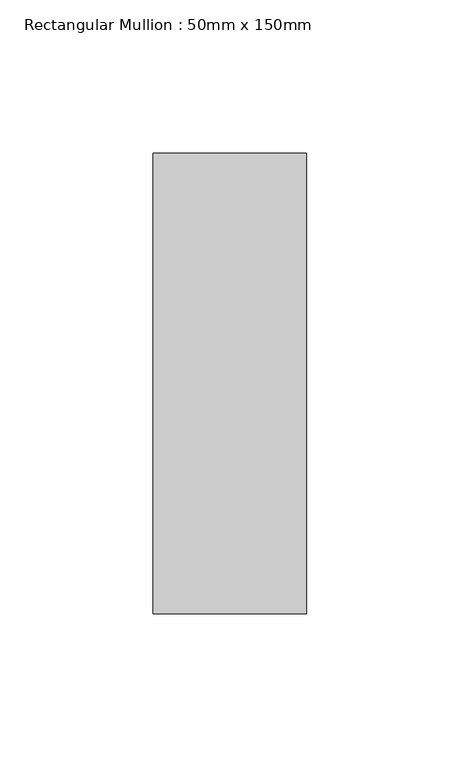
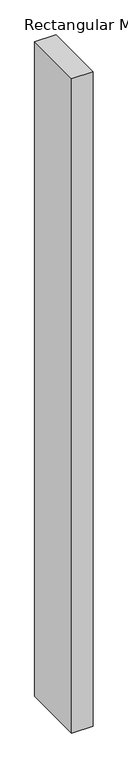
"""IFC4 building model written with IfcOpenShell, lengths in millimetres: member geometry, Rectangular Mullion : 50mm x 150mm."""

import ifcopenshell
import ifcopenshell.guid

model = None  # the IFC model being written
_history = None  # IfcOwnerHistory: only IFC2X3 demands one
_inside = {}  # id of a spatial element -> (the spatial element, [elements in it])
_under = {}  # id of a project, library or spatial element -> (it, [spatial elements below it])
_declared = {}  # id of a project -> (the project, [libraries it declares])
_typed = {}  # id of a type object -> (the type object, [elements of that type])
_made_of = {}  # id of a material, layer set ... -> (it, [elements and type objects made of it])


def new_model(schema):
    """Start an empty IFC model of exactly this schema.

    Asked for "IFC4X3", IfcOpenShell would pick the latest addendum, in which some entities
    have other attributes; the version numbers below select the first issue.
    IFC2X3 requires an IfcOwnerHistory on every rooted entity: one is made here for all.
    """
    global model, _history
    if schema == "IFC4X3":
        model = ifcopenshell.file(schema_version=(4, 3, 0, 0))
    else:
        model = ifcopenshell.file(schema=schema)
    _inside.clear()
    _under.clear()
    _declared.clear()
    _typed.clear()
    _made_of.clear()
    _history = None
    if model.schema == "IFC2X3":
        org = make("IfcOrganization", Name="unknown")
        user = make(
            "IfcPersonAndOrganization",
            ThePerson=make("IfcPerson", FamilyName="unknown"),
            TheOrganization=org,
        )
        app = make(
            "IfcApplication",
            ApplicationDeveloper=org,
            Version="unknown",
            ApplicationFullName="unknown",
            ApplicationIdentifier="unknown",
        )
        _history = make(
            "IfcOwnerHistory",
            OwningUser=user,
            OwningApplication=app,
            ChangeAction="ADDED",
            CreationDate=0,
        )
    return model


def make(cls, **values):
    """One entity of the class cls with the attributes given. An attribute that is None is left unset."""
    return model.create_entity(
        cls, **{name: value for name, value in values.items() if value is not None}
    )


def rooted(cls, **values):
    """An entity with a GlobalId (a new one), such as an element, a storey or a relation."""
    return make(cls, GlobalId=ifcopenshell.guid.new(), OwnerHistory=_history, **values)


def si_unit(unit_type, name, prefix=None):
    """IfcSIUnit, for example si_unit("LENGTHUNIT", "METRE", prefix="MILLI")."""
    return make("IfcSIUnit", UnitType=unit_type, Prefix=prefix, Name=name)


def assignment(units):
    """IfcUnitAssignment: the units of a project."""
    return None if units is None else make("IfcUnitAssignment", Units=units)


def point(xyz):
    """IfcCartesianPoint."""
    return None if xyz is None else make("IfcCartesianPoint", Coordinates=xyz)


def direction(xyz):
    """IfcDirection."""
    return None if xyz is None else make("IfcDirection", DirectionRatios=xyz)


def frame(location, z_axis=None, x_axis=None):
    """IfcAxis2Placement3D, a coordinate frame: its origin and axes. An axis left out is left unset."""
    return make(
        "IfcAxis2Placement3D",
        Location=point(location),
        Axis=direction(z_axis),
        RefDirection=direction(x_axis),
    )


def origin():
    """The frame at (0, 0, 0) with its axes left unset."""
    return frame((0.0, 0.0, 0.0))


def place(relative_to, where):
    """IfcLocalPlacement: puts the frame where relative to a parent placement (None: the world)."""
    return make(
        "IfcLocalPlacement", PlacementRelTo=relative_to, RelativePlacement=where
    )


def context(
    kind, dimensions, precision=None, world=None, true_north=None, identifier=None
):
    """IfcGeometricRepresentationContext, for example the 3D "Model" context."""
    return make(
        "IfcGeometricRepresentationContext",
        ContextIdentifier=identifier,
        ContextType=kind,
        CoordinateSpaceDimension=dimensions,
        Precision=precision,
        WorldCoordinateSystem=world,
        TrueNorth=true_north,
    )


def project(units=None, contexts=None):
    """IfcProject with its units and contexts."""
    return rooted(
        "IfcProject",
        Name="project",
        RepresentationContexts=contexts,
        UnitsInContext=assignment(units),
    )


def spatial(cls, under=None, at=None, **own):
    """A site, building, storey or space (cls), placed at a placement, below another one or the project."""
    s = rooted(cls, ObjectPlacement=at, **own)
    if under is not None:
        _under.setdefault(under.id(), (under, []))[1].append(s)
    return s


def polyline(points):
    """IfcPolyline through the points."""
    return make("IfcPolyline", Points=[point(p) for p in points])


def outline(outer, holes=None, kind="AREA"):
    """IfcArbitraryClosedProfileDef: a profile drawn as a closed curve; with holes, ...WithVoids."""
    if holes is None:
        return make("IfcArbitraryClosedProfileDef", ProfileType=kind, OuterCurve=outer)
    return make(
        "IfcArbitraryProfileDefWithVoids",
        ProfileType=kind,
        OuterCurve=outer,
        InnerCurves=holes,
    )


def extrude(swept, where, along, depth):
    """IfcExtrudedAreaSolid: the profile swept, set in the frame where, extruded along a direction by depth."""
    return make(
        "IfcExtrudedAreaSolid",
        SweptArea=swept,
        Position=where,
        ExtrudedDirection=direction(along),
        Depth=depth,
    )


def shape(context_of_items, identifier, shape_type, items):
    """IfcShapeRepresentation: the items that make up one representation, for example the "Body"."""
    return make(
        "IfcShapeRepresentation",
        ContextOfItems=context_of_items,
        RepresentationIdentifier=identifier,
        RepresentationType=shape_type,
        Items=items,
    )


def source(mapping_origin, context_of_items, identifier, shape_type, items):
    """IfcRepresentationMap: a shape defined once, which mapped items show again and again."""
    return make(
        "IfcRepresentationMap",
        MappingOrigin=mapping_origin,
        MappedRepresentation=shape(context_of_items, identifier, shape_type, items),
    )


def transform(
    local_origin,
    x_axis=None,
    y_axis=None,
    z_axis=None,
    scale=None,
    scale2=None,
    scale3=None,
    uniform=True,
):
    """IfcCartesianTransformationOperator3D, or its non-uniform kind. x_axis, y_axis, z_axis: its Axis1, 2, 3."""
    if uniform:
        return make(
            "IfcCartesianTransformationOperator3D",
            Axis1=direction(x_axis),
            Axis2=direction(y_axis),
            LocalOrigin=point(local_origin),
            Scale=scale,
            Axis3=direction(z_axis),
        )
    return make(
        "IfcCartesianTransformationOperator3DnonUniform",
        Axis1=direction(x_axis),
        Axis2=direction(y_axis),
        LocalOrigin=point(local_origin),
        Scale=scale,
        Axis3=direction(z_axis),
        Scale2=scale2,
        Scale3=scale3,
    )


def mapped(mapping_source, mapping_target):
    """IfcMappedItem: shows the shape of a source again, moved by a transform."""
    return make(
        "IfcMappedItem", MappingSource=mapping_source, MappingTarget=mapping_target
    )


def made_of(thing, what):
    """Note that an element or type object is made of a material, layer set ...; save() writes the relation."""
    if what is not None:
        _made_of.setdefault(what.id(), (what, []))[1].append(thing)
    return thing


def element(
    cls,
    number,
    at=None,
    inside=None,
    cuts=None,
    type_object=None,
    material=None,
    context=None,
    identifier="Body",
    shape_type=None,
    held_by="IfcProductDefinitionShape",
    body=None,
    shapes=None,
    **own,
):
    """One element of the class cls, such as IfcWall. Its Tag is "e" and its number.

    at: its placement. inside: the storey or other place that contains it. cuts: it is an
    opening in that element (IfcRelVoidsElement). A single representation is given by context,
    identifier, shape_type and body (its items); several are given by shapes. held_by: the class
    of the entity that holds the representations. save() writes the other relations.
    """
    e = rooted(cls, Tag="e%d" % number, ObjectPlacement=at, **own)
    if body is not None:
        shapes = [shape(context, identifier, shape_type, body)]
    if shapes is not None:
        e.Representation = make(held_by, Representations=shapes)
    if inside is not None:
        _inside.setdefault(inside.id(), (inside, []))[1].append(e)
    if cuts is not None:
        rooted(
            "IfcRelVoidsElement", RelatingBuildingElement=cuts, RelatedOpeningElement=e
        )
    if type_object is not None:
        _typed.setdefault(type_object.id(), (type_object, []))[1].append(e)
    return made_of(e, material)


def aggregate(whole, parts):
    """IfcRelAggregates: a whole, such as a stair, and the parts it consists of."""
    return rooted("IfcRelAggregates", RelatingObject=whole, RelatedObjects=parts)


def save(model, path):
    """Write the relations noted so far, then the file.

    IfcRelAggregates (storeys below a building ...), IfcRelContainedInSpatialStructure (elements
    in a storey), IfcRelDefinesByType, IfcRelAssociatesMaterial and IfcRelDeclares: one each for
    every whole, place, type object, material and project.
    """
    for whole, parts in _under.values():
        aggregate(whole, parts)
    for where, things in _inside.values():
        rooted(
            "IfcRelContainedInSpatialStructure",
            RelatedElements=things,
            RelatingStructure=where,
        )
    for kind, things in _typed.values():
        rooted("IfcRelDefinesByType", RelatedObjects=things, RelatingType=kind)
    for what, things in _made_of.values():
        rooted("IfcRelAssociatesMaterial", RelatedObjects=things, RelatingMaterial=what)
    for by, libraries in _declared.values():
        rooted("IfcRelDeclares", RelatingContext=by, RelatedDefinitions=libraries)
    model.write(path)


def rectangular_mullion_50mm_x_150mm_21b23f86(model_context):
    return source(origin(), model_context, "Body", "SweptSolid", [
        extrude(outline(polyline([(0.0, 75.0), (0.0, -75.0), (-50.0, -75.0), (-50.0, 75.0), (0.0, 75.0)])), frame((0.0, 0.0, -1615.6357052), z_axis=(0.0, 0.0, 1.0), x_axis=(1.0, 0.0, 0.0)), (0.0, 0.0, 1.0), 1615.6357052),
    ])


if __name__ == "__main__":
    model = new_model("IFC4")
    model_context = context("Model", 3, world=origin())
    ifc_project = project(units=[si_unit("LENGTHUNIT", "METRE", prefix="MILLI")], contexts=[model_context])
    site = spatial("IfcSite", under=ifc_project)
    building = spatial("IfcBuilding", under=site)
    placement = place(None, origin())
    rectangular_mullion_50mm_x_150mm_shape = rectangular_mullion_50mm_x_150mm_21b23f86(model_context)
    element("IfcMember", 1, ObjectType="Rectangular Mullion : 50mm x 150mm", at=placement, inside=building, context=model_context, shape_type="MappedRepresentation", body=[
        mapped(rectangular_mullion_50mm_x_150mm_shape, transform((0.0, 0.0, 0.0), x_axis=(1.0, 0.0, 0.0), y_axis=(0.0, 1.0, 0.0), z_axis=(0.0, 0.0, 1.0))),
    ])
    save(model, "model.ifc")

# Revit data of these elements
# Type "Rectangular Mullion : 50mm x 150mm"
#   built-in parameter 1007304 = 0.492126 (stored number, unit not read)
#   built-in parameter 1007301 = 0.082021 (stored number, unit not read)
#   built-in parameter 1007300 = 0.082021 (stored number, unit not read)
# Element 1 (IfcMember, "Rectangular Mullion : 50mm x 150mm")
#   Materials on its faces: "Aluminum"
# Materials
#   "Aluminum": class "Metal", colour RGB 244 244 244, transparency 0, Description = "Aluminum 6061", Cost = 0
